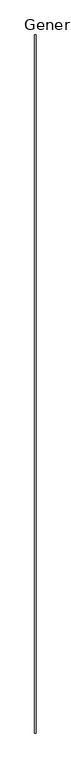
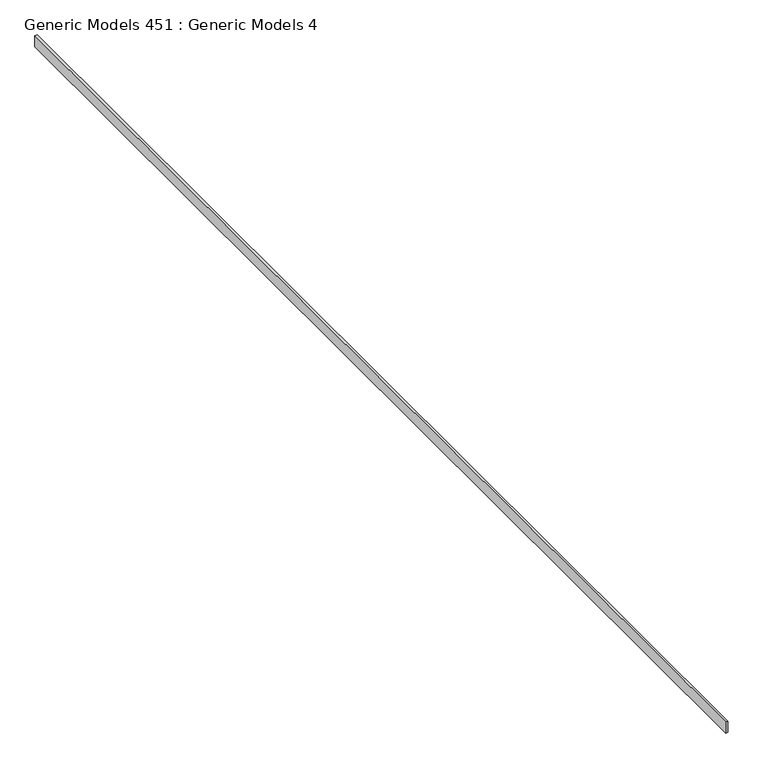
"""IFC4 building model written with IfcOpenShell, lengths in millimetres: proxy geometry, Generic Models 451 : Generic Models 4."""

from ifc_helpers import new_model, si_unit, frame, origin, place, context, project, spatial, polyline, outline, extrude, source, transform, mapped, element, save


def generic_models_451_generic_models_4_6751e52f(model_context):
    return source(origin(), model_context, "Body", "SweptSolid", [
        extrude(outline(polyline([(1555.5763704, 11855.1393978), (1580.9763704, 11855.1393978), (1580.9763704, -2064.0606022), (1555.5763704, -2064.0606022), (1555.5763704, 11855.1393978)])), frame((0.0, 0.0, 126263.146), z_axis=(0.0, 0.0, 1.0), x_axis=(1.0, 0.0, 0.0)), (0.0, 0.0, 1.0), 139.7),
    ])


if __name__ == "__main__":
    model = new_model("IFC4")
    model_context = context("Model", 3, world=origin())
    ifc_project = project(units=[si_unit("LENGTHUNIT", "METRE", prefix="MILLI")], contexts=[model_context])
    site = spatial("IfcSite", under=ifc_project)
    building = spatial("IfcBuilding", under=site)
    placement = place(None, origin())
    generic_models_451_generic_models_4_shape = generic_models_451_generic_models_4_6751e52f(model_context)
    element("IfcBuildingElementProxy", 1, Name="Generic Models 451 : Generic Models 4", ObjectType="Generic Models 451 : Generic Models 4", at=placement, inside=building, context=model_context, shape_type="MappedRepresentation", body=[
        mapped(generic_models_451_generic_models_4_shape, transform((0.0, 0.0, 0.0), x_axis=(1.0, 0.0, 0.0), y_axis=(0.0, 1.0, 0.0), z_axis=(0.0, 0.0, 1.0))),
    ])
    save(model, "model.ifc")

# Revit data of these elements
# Element 1 (IfcBuildingElementProxy, "Generic Models 451 : Generic Models 4")
#   Materials on its faces: "_STRUCTURAL MEMBER (SEE STRUCT. DWGS)"
# Materials
#   "_STRUCTURAL MEMBER (SEE STRUCT. DWGS)": class "Generic", colour RGB 209 182 141, transparency 0, Cost = 0
